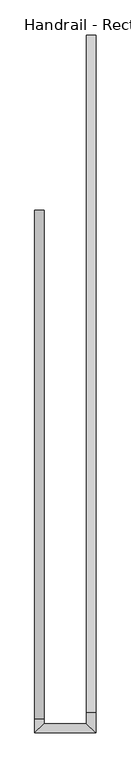
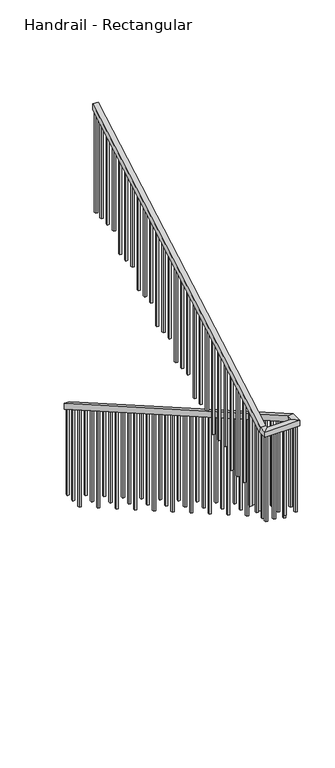
"""IFC4 building model written with IfcOpenShell, lengths in millimetres: railing geometry, Handrail - Rectangular."""

from ifc_helpers import new_model, si_unit, frame, origin, place, context, project, spatial, polyline, outline, extrude, faceted_brep, source, transform, mapped, element, save


def handrail_rectangular_4fb17f65(model_context):
    return source(origin(), model_context, "Body", "SolidModel", [
        faceted_brep([(-74520.9965, 13874.75, 13655.675), (-74470.1965, 13874.75, 13655.675), (-74470.1965, 13874.75, 13597.1285012), (-74520.9965, 13874.75, 13597.1285012), (-74520.9965, 10217.15, 15751.175), (-74470.1965, 10217.15, 15751.175), (-74470.1965, 10203.6288385, 15700.375), (-74520.9965, 10203.6288385, 15700.375), (-74520.9965, 10160.0, 15751.175), (-74470.1965, 10109.2, 15751.175), (-74470.1965, 10109.2, 15700.375), (-74520.9965, 10160.0, 15700.375), (-74749.5965, 12928.6, 17322.8), (-74749.5965, 12928.6, 17264.2535012), (-74800.3965, 12928.6, 17264.2535012), (-74800.3965, 12928.6, 17322.8), (-74800.3965, 10185.4, 15751.175), (-74749.5965, 10185.4, 15751.175), (-74800.3965, 10198.9211615, 15700.375), (-74749.5965, 10198.9211615, 15700.375), (-74749.5965, 10160.0, 15751.175), (-74800.3965, 10109.2, 15751.175), (-74800.3965, 10109.2, 15700.375), (-74749.5965, 10160.0, 15700.375)], [[[0, 1, 2, 3]], [[1, 0, 4, 5]], [[2, 1, 5, 6]], [[3, 2, 6, 7]], [[0, 3, 7, 4]], [[5, 4, 8, 9]], [[6, 5, 9, 10]], [[7, 6, 10, 11]], [[4, 7, 11, 8]], [[12, 13, 14, 15]], [[16, 17, 12, 15]], [[18, 16, 15, 14]], [[19, 18, 14, 13]], [[17, 19, 13, 12]], [[9, 8, 20, 21]], [[10, 9, 21, 22]], [[11, 10, 22, 23]], [[8, 11, 23, 20]], [[21, 20, 17, 16]], [[22, 21, 16, 18]], [[23, 22, 18, 19]], [[20, 23, 19, 17]]]),
        extrude(outline(polyline([(12817.475, 17200.5881367), (12836.525, 17211.5021992), (12836.525, 16233.775), (12817.475, 16233.775), (12817.475, 17200.5881367)])), frame((-74784.5215, 0.0, 0.0), z_axis=(1.0, 0.0, 0.0), x_axis=(0.0, 1.0, 0.0)), (0.0, 0.0, 1.0), 19.05),
        extrude(outline(polyline([(12715.875, 17142.3798033), (12734.925, 17153.2938658), (12734.925, 16233.775), (12715.875, 16233.775), (12715.875, 17142.3798033)])), frame((-74784.5215, 0.0, 0.0), z_axis=(1.0, 0.0, 0.0), x_axis=(0.0, 1.0, 0.0)), (0.0, 0.0, 1.0), 19.05),
        extrude(outline(polyline([(12614.275, 17084.17147), (12633.325, 17095.0855325), (12633.325, 16233.775), (12614.275, 16233.775), (12614.275, 17084.17147)])), frame((-74784.5215, 0.0, 0.0), z_axis=(1.0, 0.0, 0.0), x_axis=(0.0, 1.0, 0.0)), (0.0, 0.0, 1.0), 19.05),
        extrude(outline(polyline([(12512.675, 17025.9631367), (12531.725, 17036.8771992), (12531.725, 16059.15), (12512.675, 16059.15), (12512.675, 17025.9631367)])), frame((-74784.5215, 0.0, 0.0), z_axis=(1.0, 0.0, 0.0), x_axis=(0.0, 1.0, 0.0)), (0.0, 0.0, 1.0), 19.05),
        extrude(outline(polyline([(12411.075, 16967.7548033), (12430.125, 16978.6688658), (12430.125, 16059.15), (12411.075, 16059.15), (12411.075, 16967.7548033)])), frame((-74784.5215, 0.0, 0.0), z_axis=(1.0, 0.0, 0.0), x_axis=(0.0, 1.0, 0.0)), (0.0, 0.0, 1.0), 19.05),
        extrude(outline(polyline([(12309.475, 16909.54647), (12328.525, 16920.4605325), (12328.525, 16059.15), (12309.475, 16059.15), (12309.475, 16909.54647)])), frame((-74784.5215, 0.0, 0.0), z_axis=(1.0, 0.0, 0.0), x_axis=(0.0, 1.0, 0.0)), (0.0, 0.0, 1.0), 19.05),
        extrude(outline(polyline([(12207.875, 16851.3381367), (12226.925, 16862.2521992), (12226.925, 15884.525), (12207.875, 15884.525), (12207.875, 16851.3381367)])), frame((-74784.5215, 0.0, 0.0), z_axis=(1.0, 0.0, 0.0), x_axis=(0.0, 1.0, 0.0)), (0.0, 0.0, 1.0), 19.05),
        extrude(outline(polyline([(12106.275, 16793.1298033), (12125.325, 16804.0438658), (12125.325, 15884.525), (12106.275, 15884.525), (12106.275, 16793.1298033)])), frame((-74784.5215, 0.0, 0.0), z_axis=(1.0, 0.0, 0.0), x_axis=(0.0, 1.0, 0.0)), (0.0, 0.0, 1.0), 19.05),
        extrude(outline(polyline([(12004.675, 16734.92147), (12023.725, 16745.8355325), (12023.725, 15884.525), (12004.675, 15884.525), (12004.675, 16734.92147)])), frame((-74784.5215, 0.0, 0.0), z_axis=(1.0, 0.0, 0.0), x_axis=(0.0, 1.0, 0.0)), (0.0, 0.0, 1.0), 19.05),
        extrude(outline(polyline([(11903.075, 16676.7131367), (11922.125, 16687.6271992), (11922.125, 15709.9), (11903.075, 15709.9), (11903.075, 16676.7131367)])), frame((-74784.5215, 0.0, 0.0), z_axis=(1.0, 0.0, 0.0), x_axis=(0.0, 1.0, 0.0)), (0.0, 0.0, 1.0), 19.05),
        extrude(outline(polyline([(11801.475, 16618.5048033), (11820.525, 16629.4188658), (11820.525, 15709.9), (11801.475, 15709.9), (11801.475, 16618.5048033)])), frame((-74784.5215, 0.0, 0.0), z_axis=(1.0, 0.0, 0.0), x_axis=(0.0, 1.0, 0.0)), (0.0, 0.0, 1.0), 19.05),
        extrude(outline(polyline([(11699.875, 16560.29647), (11718.925, 16571.2105325), (11718.925, 15709.9), (11699.875, 15709.9), (11699.875, 16560.29647)])), frame((-74784.5215, 0.0, 0.0), z_axis=(1.0, 0.0, 0.0), x_axis=(0.0, 1.0, 0.0)), (0.0, 0.0, 1.0), 19.05),
        extrude(outline(polyline([(11598.275, 16502.0881367), (11617.325, 16513.0021992), (11617.325, 15535.275), (11598.275, 15535.275), (11598.275, 16502.0881367)])), frame((-74784.5215, 0.0, 0.0), z_axis=(1.0, 0.0, 0.0), x_axis=(0.0, 1.0, 0.0)), (0.0, 0.0, 1.0), 19.05),
        extrude(outline(polyline([(11496.675, 16443.8798033), (11515.725, 16454.7938658), (11515.725, 15535.275), (11496.675, 15535.275), (11496.675, 16443.8798033)])), frame((-74784.5215, 0.0, 0.0), z_axis=(1.0, 0.0, 0.0), x_axis=(0.0, 1.0, 0.0)), (0.0, 0.0, 1.0), 19.05),
        extrude(outline(polyline([(11395.075, 16385.67147), (11414.125, 16396.5855325), (11414.125, 15535.275), (11395.075, 15535.275), (11395.075, 16385.67147)])), frame((-74784.5215, 0.0, 0.0), z_axis=(1.0, 0.0, 0.0), x_axis=(0.0, 1.0, 0.0)), (0.0, 0.0, 1.0), 19.05),
        extrude(outline(polyline([(11293.475, 16327.4631367), (11312.525, 16338.3771992), (11312.525, 15360.65), (11293.475, 15360.65), (11293.475, 16327.4631367)])), frame((-74784.5215, 0.0, 0.0), z_axis=(1.0, 0.0, 0.0), x_axis=(0.0, 1.0, 0.0)), (0.0, 0.0, 1.0), 19.05),
        extrude(outline(polyline([(11191.875, 16269.2548033), (11210.925, 16280.1688658), (11210.925, 15360.65), (11191.875, 15360.65), (11191.875, 16269.2548033)])), frame((-74784.5215, 0.0, 0.0), z_axis=(1.0, 0.0, 0.0), x_axis=(0.0, 1.0, 0.0)), (0.0, 0.0, 1.0), 19.05),
        extrude(outline(polyline([(11090.275, 16211.04647), (11109.325, 16221.9605325), (11109.325, 15360.65), (11090.275, 15360.65), (11090.275, 16211.04647)])), frame((-74784.5215, 0.0, 0.0), z_axis=(1.0, 0.0, 0.0), x_axis=(0.0, 1.0, 0.0)), (0.0, 0.0, 1.0), 19.05),
        extrude(outline(polyline([(10988.675, 16152.8381367), (11007.725, 16163.7521992), (11007.725, 15186.025), (10988.675, 15186.025), (10988.675, 16152.8381367)])), frame((-74784.5215, 0.0, 0.0), z_axis=(1.0, 0.0, 0.0), x_axis=(0.0, 1.0, 0.0)), (0.0, 0.0, 1.0), 19.05),
        extrude(outline(polyline([(10887.075, 16094.6298033), (10906.125, 16105.5438658), (10906.125, 15186.025), (10887.075, 15186.025), (10887.075, 16094.6298033)])), frame((-74784.5215, 0.0, 0.0), z_axis=(1.0, 0.0, 0.0), x_axis=(0.0, 1.0, 0.0)), (0.0, 0.0, 1.0), 19.05),
        extrude(outline(polyline([(10785.475, 16036.42147), (10804.525, 16047.3355325), (10804.525, 15186.025), (10785.475, 15186.025), (10785.475, 16036.42147)])), frame((-74784.5215, 0.0, 0.0), z_axis=(1.0, 0.0, 0.0), x_axis=(0.0, 1.0, 0.0)), (0.0, 0.0, 1.0), 19.05),
        extrude(outline(polyline([(10683.875, 15978.2131367), (10702.925, 15989.1271992), (10702.925, 15011.4), (10683.875, 15011.4), (10683.875, 15978.2131367)])), frame((-74784.5215, 0.0, 0.0), z_axis=(1.0, 0.0, 0.0), x_axis=(0.0, 1.0, 0.0)), (0.0, 0.0, 1.0), 19.05),
        extrude(outline(polyline([(10582.275, 15920.0048033), (10601.325, 15930.9188658), (10601.325, 15011.4), (10582.275, 15011.4), (10582.275, 15920.0048033)])), frame((-74784.5215, 0.0, 0.0), z_axis=(1.0, 0.0, 0.0), x_axis=(0.0, 1.0, 0.0)), (0.0, 0.0, 1.0), 19.05),
        extrude(outline(polyline([(10480.675, 15861.79647), (10499.725, 15872.7105325), (10499.725, 15011.4), (10480.675, 15011.4), (10480.675, 15861.79647)])), frame((-74784.5215, 0.0, 0.0), z_axis=(1.0, 0.0, 0.0), x_axis=(0.0, 1.0, 0.0)), (0.0, 0.0, 1.0), 19.05),
        extrude(outline(polyline([(10379.075, 15803.5881367), (10398.125, 15814.5021992), (10398.125, 14836.775), (10379.075, 14836.775), (10379.075, 15803.5881367)])), frame((-74784.5215, 0.0, 0.0), z_axis=(1.0, 0.0, 0.0), x_axis=(0.0, 1.0, 0.0)), (0.0, 0.0, 1.0), 19.05),
        extrude(outline(polyline([(10277.475, 15745.3798033), (10296.525, 15756.2938658), (10296.525, 14836.775), (10277.475, 14836.775), (10277.475, 15745.3798033)])), frame((-74784.5215, 0.0, 0.0), z_axis=(1.0, 0.0, 0.0), x_axis=(0.0, 1.0, 0.0)), (0.0, 0.0, 1.0), 19.05),
        extrude(outline(polyline([(-74689.2715, 10144.125), (-74689.2715, 10125.075), (-74708.3215, 10125.075), (-74708.3215, 10144.125), (-74689.2715, 10144.125)])), frame((0.0, 0.0, 14836.775), z_axis=(0.0, 0.0, 1.0), x_axis=(1.0, 0.0, 0.0)), (0.0, 0.0, 1.0), 863.6),
        extrude(outline(polyline([(-74587.6715, 10144.125), (-74587.6715, 10125.075), (-74606.7215, 10125.075), (-74606.7215, 10144.125), (-74587.6715, 10144.125)])), frame((0.0, 0.0, 14836.775), z_axis=(0.0, 0.0, 1.0), x_axis=(1.0, 0.0, 0.0)), (0.0, 0.0, 1.0), 863.6),
        extrude(outline(polyline([(10309.225, 15639.8771992), (10328.275, 15628.9631367), (10328.275, 14662.15), (10309.225, 14662.15), (10309.225, 15639.8771992)])), frame((-74505.1215, 0.0, 0.0), z_axis=(1.0, 0.0, 0.0), x_axis=(0.0, 1.0, 0.0)), (0.0, 0.0, 1.0), 19.05),
        extrude(outline(polyline([(10410.825, 15581.6688658), (10429.875, 15570.7548033), (10429.875, 14662.15), (10410.825, 14662.15), (10410.825, 15581.6688658)])), frame((-74505.1215, 0.0, 0.0), z_axis=(1.0, 0.0, 0.0), x_axis=(0.0, 1.0, 0.0)), (0.0, 0.0, 1.0), 19.05),
        extrude(outline(polyline([(10512.425, 15523.4605325), (10531.475, 15512.54647), (10531.475, 14662.15), (10512.425, 14662.15), (10512.425, 15523.4605325)])), frame((-74505.1215, 0.0, 0.0), z_axis=(1.0, 0.0, 0.0), x_axis=(0.0, 1.0, 0.0)), (0.0, 0.0, 1.0), 19.05),
        extrude(outline(polyline([(10614.025, 15465.2521992), (10633.075, 15454.3381367), (10633.075, 14487.525), (10614.025, 14487.525), (10614.025, 15465.2521992)])), frame((-74505.1215, 0.0, 0.0), z_axis=(1.0, 0.0, 0.0), x_axis=(0.0, 1.0, 0.0)), (0.0, 0.0, 1.0), 19.05),
        extrude(outline(polyline([(10715.625, 15407.0438658), (10734.675, 15396.1298033), (10734.675, 14487.525), (10715.625, 14487.525), (10715.625, 15407.0438658)])), frame((-74505.1215, 0.0, 0.0), z_axis=(1.0, 0.0, 0.0), x_axis=(0.0, 1.0, 0.0)), (0.0, 0.0, 1.0), 19.05),
        extrude(outline(polyline([(10817.225, 15348.8355325), (10836.275, 15337.92147), (10836.275, 14487.525), (10817.225, 14487.525), (10817.225, 15348.8355325)])), frame((-74505.1215, 0.0, 0.0), z_axis=(1.0, 0.0, 0.0), x_axis=(0.0, 1.0, 0.0)), (0.0, 0.0, 1.0), 19.05),
        extrude(outline(polyline([(10918.825, 15290.6271992), (10937.875, 15279.7131367), (10937.875, 14312.9), (10918.825, 14312.9), (10918.825, 15290.6271992)])), frame((-74505.1215, 0.0, 0.0), z_axis=(1.0, 0.0, 0.0), x_axis=(0.0, 1.0, 0.0)), (0.0, 0.0, 1.0), 19.05),
        extrude(outline(polyline([(11020.425, 15232.4188658), (11039.475, 15221.5048033), (11039.475, 14312.9), (11020.425, 14312.9), (11020.425, 15232.4188658)])), frame((-74505.1215, 0.0, 0.0), z_axis=(1.0, 0.0, 0.0), x_axis=(0.0, 1.0, 0.0)), (0.0, 0.0, 1.0), 19.05),
        extrude(outline(polyline([(11122.025, 15174.2105325), (11141.075, 15163.29647), (11141.075, 14312.9), (11122.025, 14312.9), (11122.025, 15174.2105325)])), frame((-74505.1215, 0.0, 0.0), z_axis=(1.0, 0.0, 0.0), x_axis=(0.0, 1.0, 0.0)), (0.0, 0.0, 1.0), 19.05),
        extrude(outline(polyline([(11223.625, 15116.0021992), (11242.675, 15105.0881367), (11242.675, 14138.275), (11223.625, 14138.275), (11223.625, 15116.0021992)])), frame((-74505.1215, 0.0, 0.0), z_axis=(1.0, 0.0, 0.0), x_axis=(0.0, 1.0, 0.0)), (0.0, 0.0, 1.0), 19.05),
        extrude(outline(polyline([(11325.225, 15057.7938658), (11344.275, 15046.8798033), (11344.275, 14138.275), (11325.225, 14138.275), (11325.225, 15057.7938658)])), frame((-74505.1215, 0.0, 0.0), z_axis=(1.0, 0.0, 0.0), x_axis=(0.0, 1.0, 0.0)), (0.0, 0.0, 1.0), 19.05),
        extrude(outline(polyline([(11426.825, 14999.5855325), (11445.875, 14988.67147), (11445.875, 14138.275), (11426.825, 14138.275), (11426.825, 14999.5855325)])), frame((-74505.1215, 0.0, 0.0), z_axis=(1.0, 0.0, 0.0), x_axis=(0.0, 1.0, 0.0)), (0.0, 0.0, 1.0), 19.05),
        extrude(outline(polyline([(11528.425, 14941.3771992), (11547.475, 14930.4631367), (11547.475, 13963.65), (11528.425, 13963.65), (11528.425, 14941.3771992)])), frame((-74505.1215, 0.0, 0.0), z_axis=(1.0, 0.0, 0.0), x_axis=(0.0, 1.0, 0.0)), (0.0, 0.0, 1.0), 19.05),
        extrude(outline(polyline([(11630.025, 14883.1688658), (11649.075, 14872.2548033), (11649.075, 13963.65), (11630.025, 13963.65), (11630.025, 14883.1688658)])), frame((-74505.1215, 0.0, 0.0), z_axis=(1.0, 0.0, 0.0), x_axis=(0.0, 1.0, 0.0)), (0.0, 0.0, 1.0), 19.05),
        extrude(outline(polyline([(11731.625, 14824.9605325), (11750.675, 14814.04647), (11750.675, 13963.65), (11731.625, 13963.65), (11731.625, 14824.9605325)])), frame((-74505.1215, 0.0, 0.0), z_axis=(1.0, 0.0, 0.0), x_axis=(0.0, 1.0, 0.0)), (0.0, 0.0, 1.0), 19.05),
        extrude(outline(polyline([(11833.225, 14766.7521992), (11852.275, 14755.8381367), (11852.275, 13789.025), (11833.225, 13789.025), (11833.225, 14766.7521992)])), frame((-74505.1215, 0.0, 0.0), z_axis=(1.0, 0.0, 0.0), x_axis=(0.0, 1.0, 0.0)), (0.0, 0.0, 1.0), 19.05),
        extrude(outline(polyline([(11934.825, 14708.5438658), (11953.875, 14697.6298033), (11953.875, 13789.025), (11934.825, 13789.025), (11934.825, 14708.5438658)])), frame((-74505.1215, 0.0, 0.0), z_axis=(1.0, 0.0, 0.0), x_axis=(0.0, 1.0, 0.0)), (0.0, 0.0, 1.0), 19.05),
        extrude(outline(polyline([(12036.425, 14650.3355325), (12055.475, 14639.42147), (12055.475, 13789.025), (12036.425, 13789.025), (12036.425, 14650.3355325)])), frame((-74505.1215, 0.0, 0.0), z_axis=(1.0, 0.0, 0.0), x_axis=(0.0, 1.0, 0.0)), (0.0, 0.0, 1.0), 19.05),
        extrude(outline(polyline([(12138.025, 14592.1271992), (12157.075, 14581.2131367), (12157.075, 13614.4), (12138.025, 13614.4), (12138.025, 14592.1271992)])), frame((-74505.1215, 0.0, 0.0), z_axis=(1.0, 0.0, 0.0), x_axis=(0.0, 1.0, 0.0)), (0.0, 0.0, 1.0), 19.05),
        extrude(outline(polyline([(12239.625, 14533.9188658), (12258.675, 14523.0048033), (12258.675, 13614.4), (12239.625, 13614.4), (12239.625, 14533.9188658)])), frame((-74505.1215, 0.0, 0.0), z_axis=(1.0, 0.0, 0.0), x_axis=(0.0, 1.0, 0.0)), (0.0, 0.0, 1.0), 19.05),
        extrude(outline(polyline([(12341.225, 14475.7105325), (12360.275, 14464.79647), (12360.275, 13614.4), (12341.225, 13614.4), (12341.225, 14475.7105325)])), frame((-74505.1215, 0.0, 0.0), z_axis=(1.0, 0.0, 0.0), x_axis=(0.0, 1.0, 0.0)), (0.0, 0.0, 1.0), 19.05),
        extrude(outline(polyline([(12442.825, 14417.5021992), (12461.875, 14406.5881367), (12461.875, 13439.775), (12442.825, 13439.775), (12442.825, 14417.5021992)])), frame((-74505.1215, 0.0, 0.0), z_axis=(1.0, 0.0, 0.0), x_axis=(0.0, 1.0, 0.0)), (0.0, 0.0, 1.0), 19.05),
        extrude(outline(polyline([(12544.425, 14359.2938658), (12563.475, 14348.3798033), (12563.475, 13439.775), (12544.425, 13439.775), (12544.425, 14359.2938658)])), frame((-74505.1215, 0.0, 0.0), z_axis=(1.0, 0.0, 0.0), x_axis=(0.0, 1.0, 0.0)), (0.0, 0.0, 1.0), 19.05),
        extrude(outline(polyline([(12646.025, 14301.0855325), (12665.075, 14290.17147), (12665.075, 13439.775), (12646.025, 13439.775), (12646.025, 14301.0855325)])), frame((-74505.1215, 0.0, 0.0), z_axis=(1.0, 0.0, 0.0), x_axis=(0.0, 1.0, 0.0)), (0.0, 0.0, 1.0), 19.05),
        extrude(outline(polyline([(12747.625, 14242.8771992), (12766.675, 14231.9631367), (12766.675, 13265.15), (12747.625, 13265.15), (12747.625, 14242.8771992)])), frame((-74505.1215, 0.0, 0.0), z_axis=(1.0, 0.0, 0.0), x_axis=(0.0, 1.0, 0.0)), (0.0, 0.0, 1.0), 19.05),
        extrude(outline(polyline([(12849.225, 14184.6688658), (12868.275, 14173.7548033), (12868.275, 13265.15), (12849.225, 13265.15), (12849.225, 14184.6688658)])), frame((-74505.1215, 0.0, 0.0), z_axis=(1.0, 0.0, 0.0), x_axis=(0.0, 1.0, 0.0)), (0.0, 0.0, 1.0), 19.05),
        extrude(outline(polyline([(12950.825, 14126.4605325), (12969.875, 14115.54647), (12969.875, 13265.15), (12950.825, 13265.15), (12950.825, 14126.4605325)])), frame((-74505.1215, 0.0, 0.0), z_axis=(1.0, 0.0, 0.0), x_axis=(0.0, 1.0, 0.0)), (0.0, 0.0, 1.0), 19.05),
        extrude(outline(polyline([(13052.425, 14068.2521992), (13071.475, 14057.3381367), (13071.475, 13090.525), (13052.425, 13090.525), (13052.425, 14068.2521992)])), frame((-74505.1215, 0.0, 0.0), z_axis=(1.0, 0.0, 0.0), x_axis=(0.0, 1.0, 0.0)), (0.0, 0.0, 1.0), 19.05),
        extrude(outline(polyline([(13154.025, 14010.0438658), (13173.075, 13999.1298033), (13173.075, 13090.525), (13154.025, 13090.525), (13154.025, 14010.0438658)])), frame((-74505.1215, 0.0, 0.0), z_axis=(1.0, 0.0, 0.0), x_axis=(0.0, 1.0, 0.0)), (0.0, 0.0, 1.0), 19.05),
        extrude(outline(polyline([(13255.625, 13951.8355325), (13274.675, 13940.92147), (13274.675, 13090.525), (13255.625, 13090.525), (13255.625, 13951.8355325)])), frame((-74505.1215, 0.0, 0.0), z_axis=(1.0, 0.0, 0.0), x_axis=(0.0, 1.0, 0.0)), (0.0, 0.0, 1.0), 19.05),
        extrude(outline(polyline([(13357.225, 13893.6271992), (13376.275, 13882.7131367), (13376.275, 12915.9), (13357.225, 12915.9), (13357.225, 13893.6271992)])), frame((-74505.1215, 0.0, 0.0), z_axis=(1.0, 0.0, 0.0), x_axis=(0.0, 1.0, 0.0)), (0.0, 0.0, 1.0), 19.05),
        extrude(outline(polyline([(13458.825, 13835.4188658), (13477.875, 13824.5048033), (13477.875, 12915.9), (13458.825, 12915.9), (13458.825, 13835.4188658)])), frame((-74505.1215, 0.0, 0.0), z_axis=(1.0, 0.0, 0.0), x_axis=(0.0, 1.0, 0.0)), (0.0, 0.0, 1.0), 19.05),
        extrude(outline(polyline([(13560.425, 13777.2105325), (13579.475, 13766.29647), (13579.475, 12915.9), (13560.425, 12915.9), (13560.425, 13777.2105325)])), frame((-74505.1215, 0.0, 0.0), z_axis=(1.0, 0.0, 0.0), x_axis=(0.0, 1.0, 0.0)), (0.0, 0.0, 1.0), 19.05),
        extrude(outline(polyline([(13662.025, 13719.0021992), (13681.075, 13708.0881367), (13681.075, 12741.275), (13662.025, 12741.275), (13662.025, 13719.0021992)])), frame((-74505.1215, 0.0, 0.0), z_axis=(1.0, 0.0, 0.0), x_axis=(0.0, 1.0, 0.0)), (0.0, 0.0, 1.0), 19.05),
        extrude(outline(polyline([(13763.625, 13660.7938658), (13782.675, 13649.8798033), (13782.675, 12741.275), (13763.625, 12741.275), (13763.625, 13660.7938658)])), frame((-74505.1215, 0.0, 0.0), z_axis=(1.0, 0.0, 0.0), x_axis=(0.0, 1.0, 0.0)), (0.0, 0.0, 1.0), 19.05),
        extrude(outline(polyline([(-74765.4715, 10175.875), (-74784.5215, 10175.875), (-74784.5215, 10194.925), (-74765.4715, 10194.925), (-74765.4715, 10175.875)])), frame((0.0, 0.0, 14836.775), z_axis=(0.0, 0.0, 1.0), x_axis=(1.0, 0.0, 0.0)), (0.0, 0.0, 1.0), 863.6),
        extrude(outline(polyline([(-74765.4715, 10144.125), (-74765.4715, 10125.075), (-74784.5215, 10125.075), (-74784.5215, 10144.125), (-74765.4715, 10144.125)])), frame((0.0, 0.0, 14836.775), z_axis=(0.0, 0.0, 1.0), x_axis=(1.0, 0.0, 0.0)), (0.0, 0.0, 1.0), 863.6),
        extrude(outline(polyline([(-74505.1215, 10144.125), (-74486.0715, 10144.125), (-74486.0715, 10125.075), (-74505.1215, 10125.075), (-74505.1215, 10144.125)])), frame((0.0, 0.0, 14836.775), z_axis=(0.0, 0.0, 1.0), x_axis=(1.0, 0.0, 0.0)), (0.0, 0.0, 1.0), 863.6),
        extrude(outline(polyline([(-74505.1215, 10226.675), (-74486.0715, 10226.675), (-74486.0715, 10207.625), (-74505.1215, 10207.625), (-74505.1215, 10226.675)])), frame((0.0, 0.0, 14836.775), z_axis=(0.0, 0.0, 1.0), x_axis=(1.0, 0.0, 0.0)), (0.0, 0.0, 1.0), 863.6),
        extrude(outline(polyline([(12909.55, 17253.3394387), (12928.6, 17264.2535012), (12928.6, 16233.775), (12909.55, 16233.775), (12909.55, 17253.3394387)])), frame((-74784.5215, 0.0, 0.0), z_axis=(1.0, 0.0, 0.0), x_axis=(0.0, 1.0, 0.0)), (0.0, 0.0, 1.0), 19.05),
        extrude(outline(polyline([(13855.7, 13608.0425637), (13874.75, 13597.1285012), (13874.75, 12741.275), (13855.7, 12741.275), (13855.7, 13608.0425637)])), frame((-74505.1215, 0.0, 0.0), z_axis=(1.0, 0.0, 0.0), x_axis=(0.0, 1.0, 0.0)), (0.0, 0.0, 1.0), 19.05),
    ])


if __name__ == "__main__":
    model = new_model("IFC4")
    model_context = context("Model", 3, world=origin())
    ifc_project = project(units=[si_unit("LENGTHUNIT", "METRE", prefix="MILLI")], contexts=[model_context])
    site = spatial("IfcSite", under=ifc_project)
    building = spatial("IfcBuilding", under=site)
    placement = place(None, origin())
    handrail_rectangular_shape = handrail_rectangular_4fb17f65(model_context)
    element("IfcRailing", 1, ObjectType="Handrail - Rectangular", at=placement, inside=building, context=model_context, shape_type="MappedRepresentation", body=[
        mapped(handrail_rectangular_shape, transform((0.0, 0.0, 0.0), x_axis=(1.0, 0.0, 0.0), y_axis=(0.0, 1.0, 0.0), z_axis=(0.0, 0.0, 1.0))),
    ])
    save(model, "model.ifc")
